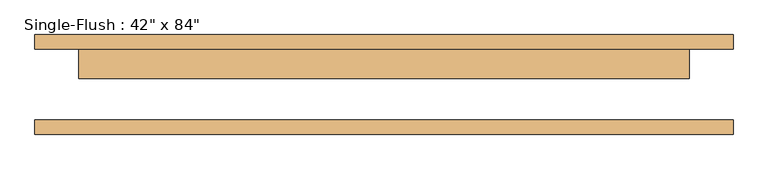
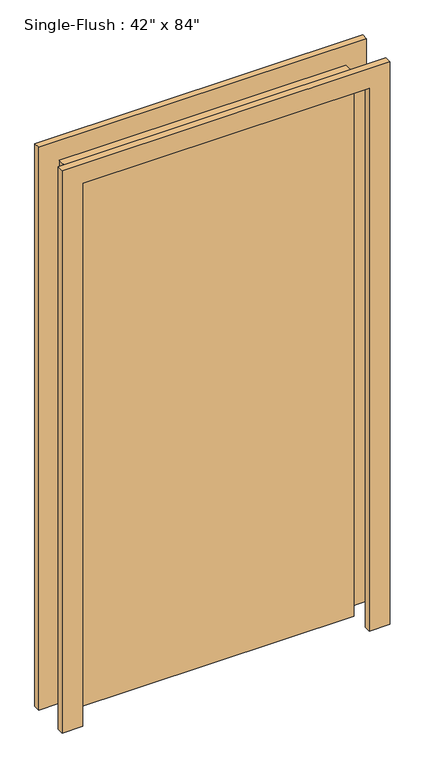
"""IFC4 building model written with IfcOpenShell, lengths in millimetres: door geometry."""

import ifcopenshell
import ifcopenshell.guid

model = None  # the IFC model being written
_history = None  # IfcOwnerHistory: only IFC2X3 demands one
_inside = {}  # id of a spatial element -> (the spatial element, [elements in it])
_under = {}  # id of a project, library or spatial element -> (it, [spatial elements below it])
_declared = {}  # id of a project -> (the project, [libraries it declares])
_typed = {}  # id of a type object -> (the type object, [elements of that type])
_made_of = {}  # id of a material, layer set ... -> (it, [elements and type objects made of it])


def new_model(schema):
    """Start an empty IFC model of exactly this schema.

    Asked for "IFC4X3", IfcOpenShell would pick the latest addendum, in which some entities
    have other attributes; the version numbers below select the first issue.
    IFC2X3 requires an IfcOwnerHistory on every rooted entity: one is made here for all.
    """
    global model, _history
    if schema == "IFC4X3":
        model = ifcopenshell.file(schema_version=(4, 3, 0, 0))
    else:
        model = ifcopenshell.file(schema=schema)
    _inside.clear()
    _under.clear()
    _declared.clear()
    _typed.clear()
    _made_of.clear()
    _history = None
    if model.schema == "IFC2X3":
        org = make("IfcOrganization", Name="unknown")
        user = make(
            "IfcPersonAndOrganization",
            ThePerson=make("IfcPerson", FamilyName="unknown"),
            TheOrganization=org,
        )
        app = make(
            "IfcApplication",
            ApplicationDeveloper=org,
            Version="unknown",
            ApplicationFullName="unknown",
            ApplicationIdentifier="unknown",
        )
        _history = make(
            "IfcOwnerHistory",
            OwningUser=user,
            OwningApplication=app,
            ChangeAction="ADDED",
            CreationDate=0,
        )
    return model


def make(cls, **values):
    """One entity of the class cls with the attributes given. An attribute that is None is left unset."""
    return model.create_entity(
        cls, **{name: value for name, value in values.items() if value is not None}
    )


def rooted(cls, **values):
    """An entity with a GlobalId (a new one), such as an element, a storey or a relation."""
    return make(cls, GlobalId=ifcopenshell.guid.new(), OwnerHistory=_history, **values)


def si_unit(unit_type, name, prefix=None):
    """IfcSIUnit, for example si_unit("LENGTHUNIT", "METRE", prefix="MILLI")."""
    return make("IfcSIUnit", UnitType=unit_type, Prefix=prefix, Name=name)


def assignment(units):
    """IfcUnitAssignment: the units of a project."""
    return None if units is None else make("IfcUnitAssignment", Units=units)


def point(xyz):
    """IfcCartesianPoint."""
    return None if xyz is None else make("IfcCartesianPoint", Coordinates=xyz)


def direction(xyz):
    """IfcDirection."""
    return None if xyz is None else make("IfcDirection", DirectionRatios=xyz)


def frame(location, z_axis=None, x_axis=None):
    """IfcAxis2Placement3D, a coordinate frame: its origin and axes. An axis left out is left unset."""
    return make(
        "IfcAxis2Placement3D",
        Location=point(location),
        Axis=direction(z_axis),
        RefDirection=direction(x_axis),
    )


def origin():
    """The frame at (0, 0, 0) with its axes left unset."""
    return frame((0.0, 0.0, 0.0))


def origin_with_axes():
    """The frame at (0, 0, 0) with the z axis (0, 0, 1) and the x axis (1, 0, 0) written out."""
    return frame((0.0, 0.0, 0.0), z_axis=(0.0, 0.0, 1.0), x_axis=(1.0, 0.0, 0.0))


def place(relative_to, where):
    """IfcLocalPlacement: puts the frame where relative to a parent placement (None: the world)."""
    return make(
        "IfcLocalPlacement", PlacementRelTo=relative_to, RelativePlacement=where
    )


def context(
    kind, dimensions, precision=None, world=None, true_north=None, identifier=None
):
    """IfcGeometricRepresentationContext, for example the 3D "Model" context."""
    return make(
        "IfcGeometricRepresentationContext",
        ContextIdentifier=identifier,
        ContextType=kind,
        CoordinateSpaceDimension=dimensions,
        Precision=precision,
        WorldCoordinateSystem=world,
        TrueNorth=true_north,
    )


def project(units=None, contexts=None):
    """IfcProject with its units and contexts."""
    return rooted(
        "IfcProject",
        Name="project",
        RepresentationContexts=contexts,
        UnitsInContext=assignment(units),
    )


def spatial(cls, under=None, at=None, **own):
    """A site, building, storey or space (cls), placed at a placement, below another one or the project."""
    s = rooted(cls, ObjectPlacement=at, **own)
    if under is not None:
        _under.setdefault(under.id(), (under, []))[1].append(s)
    return s


def polyline(points):
    """IfcPolyline through the points."""
    return make("IfcPolyline", Points=[point(p) for p in points])


def outline(outer, holes=None, kind="AREA"):
    """IfcArbitraryClosedProfileDef: a profile drawn as a closed curve; with holes, ...WithVoids."""
    if holes is None:
        return make("IfcArbitraryClosedProfileDef", ProfileType=kind, OuterCurve=outer)
    return make(
        "IfcArbitraryProfileDefWithVoids",
        ProfileType=kind,
        OuterCurve=outer,
        InnerCurves=holes,
    )


def extrude(swept, where, along, depth):
    """IfcExtrudedAreaSolid: the profile swept, set in the frame where, extruded along a direction by depth."""
    return make(
        "IfcExtrudedAreaSolid",
        SweptArea=swept,
        Position=where,
        ExtrudedDirection=direction(along),
        Depth=depth,
    )


def shape(context_of_items, identifier, shape_type, items):
    """IfcShapeRepresentation: the items that make up one representation, for example the "Body"."""
    return make(
        "IfcShapeRepresentation",
        ContextOfItems=context_of_items,
        RepresentationIdentifier=identifier,
        RepresentationType=shape_type,
        Items=items,
    )


def source(mapping_origin, context_of_items, identifier, shape_type, items):
    """IfcRepresentationMap: a shape defined once, which mapped items show again and again."""
    return make(
        "IfcRepresentationMap",
        MappingOrigin=mapping_origin,
        MappedRepresentation=shape(context_of_items, identifier, shape_type, items),
    )


def transform(
    local_origin,
    x_axis=None,
    y_axis=None,
    z_axis=None,
    scale=None,
    scale2=None,
    scale3=None,
    uniform=True,
):
    """IfcCartesianTransformationOperator3D, or its non-uniform kind. x_axis, y_axis, z_axis: its Axis1, 2, 3."""
    if uniform:
        return make(
            "IfcCartesianTransformationOperator3D",
            Axis1=direction(x_axis),
            Axis2=direction(y_axis),
            LocalOrigin=point(local_origin),
            Scale=scale,
            Axis3=direction(z_axis),
        )
    return make(
        "IfcCartesianTransformationOperator3DnonUniform",
        Axis1=direction(x_axis),
        Axis2=direction(y_axis),
        LocalOrigin=point(local_origin),
        Scale=scale,
        Axis3=direction(z_axis),
        Scale2=scale2,
        Scale3=scale3,
    )


def mapped(mapping_source, mapping_target):
    """IfcMappedItem: shows the shape of a source again, moved by a transform."""
    return make(
        "IfcMappedItem", MappingSource=mapping_source, MappingTarget=mapping_target
    )


def made_of(thing, what):
    """Note that an element or type object is made of a material, layer set ...; save() writes the relation."""
    if what is not None:
        _made_of.setdefault(what.id(), (what, []))[1].append(thing)
    return thing


def element(
    cls,
    number,
    at=None,
    inside=None,
    cuts=None,
    type_object=None,
    material=None,
    context=None,
    identifier="Body",
    shape_type=None,
    held_by="IfcProductDefinitionShape",
    body=None,
    shapes=None,
    **own,
):
    """One element of the class cls, such as IfcWall. Its Tag is "e" and its number.

    at: its placement. inside: the storey or other place that contains it. cuts: it is an
    opening in that element (IfcRelVoidsElement). A single representation is given by context,
    identifier, shape_type and body (its items); several are given by shapes. held_by: the class
    of the entity that holds the representations. save() writes the other relations.
    """
    e = rooted(cls, Tag="e%d" % number, ObjectPlacement=at, **own)
    if body is not None:
        shapes = [shape(context, identifier, shape_type, body)]
    if shapes is not None:
        e.Representation = make(held_by, Representations=shapes)
    if inside is not None:
        _inside.setdefault(inside.id(), (inside, []))[1].append(e)
    if cuts is not None:
        rooted(
            "IfcRelVoidsElement", RelatingBuildingElement=cuts, RelatedOpeningElement=e
        )
    if type_object is not None:
        _typed.setdefault(type_object.id(), (type_object, []))[1].append(e)
    return made_of(e, material)


def aggregate(whole, parts):
    """IfcRelAggregates: a whole, such as a stair, and the parts it consists of."""
    return rooted("IfcRelAggregates", RelatingObject=whole, RelatedObjects=parts)


def save(model, path):
    """Write the relations noted so far, then the file.

    IfcRelAggregates (storeys below a building ...), IfcRelContainedInSpatialStructure (elements
    in a storey), IfcRelDefinesByType, IfcRelAssociatesMaterial and IfcRelDeclares: one each for
    every whole, place, type object, material and project.
    """
    for whole, parts in _under.values():
        aggregate(whole, parts)
    for where, things in _inside.values():
        rooted(
            "IfcRelContainedInSpatialStructure",
            RelatedElements=things,
            RelatingStructure=where,
        )
    for kind, things in _typed.values():
        rooted("IfcRelDefinesByType", RelatedObjects=things, RelatingType=kind)
    for what, things in _made_of.values():
        rooted("IfcRelAssociatesMaterial", RelatedObjects=things, RelatingMaterial=what)
    for by, libraries in _declared.values():
        rooted("IfcRelDeclares", RelatingContext=by, RelatedDefinitions=libraries)
    model.write(path)


def door_af0cb62c(model_context):
    return source(origin(), model_context, "Body", "SweptSolid", [
        extrude(outline(polyline([(2209.8, -609.6), (0.0, -609.6), (0.0, -533.4), (2133.6, -533.4), (2133.6, 533.4), (0.0, 533.4), (0.0, 609.6), (2209.8, 609.6), (2209.8, -609.6)])), frame((0.0, 61.9125, 0.0), z_axis=(0.0, 1.0, 0.0), x_axis=(0.0, 0.0, 1.0)), (0.0, 0.0, 1.0), 25.4),
        extrude(outline(polyline([(2209.8, 609.6), (2209.8, -609.6), (0.0, -609.6), (0.0, -533.4), (2133.6, -533.4), (2133.6, 533.4), (0.0, 533.4), (0.0, 609.6), (2209.8, 609.6)])), frame((0.0, -87.3125, 0.0), z_axis=(0.0, 1.0, 0.0), x_axis=(0.0, 0.0, 1.0)), (0.0, 0.0, 1.0), 25.4),
        extrude(outline(polyline([(533.4, 11.1125), (-533.4, 11.1125), (-533.4, 61.9125), (533.4, 61.9125), (533.4, 11.1125)])), origin_with_axes(), (0.0, 0.0, 1.0), 2133.6),
    ])


if __name__ == "__main__":
    model = new_model("IFC4")
    model_context = context("Model", 3, world=origin())
    ifc_project = project(units=[si_unit("LENGTHUNIT", "METRE", prefix="MILLI")], contexts=[model_context])
    site = spatial("IfcSite", under=ifc_project)
    building = spatial("IfcBuilding", under=site)
    placement = place(None, origin())
    door_shape = door_af0cb62c(model_context)
    element("IfcDoor", 1, ObjectType="Single-Flush : 42\" x 84\"", at=placement, inside=building, context=model_context, shape_type="MappedRepresentation", body=[
        mapped(door_shape, transform((0.0, 0.0, 0.0), x_axis=(1.0, 0.0, 0.0), y_axis=(0.0, 1.0, 0.0), z_axis=(0.0, 0.0, 1.0))),
    ])
    save(model, "model.ifc")

# Revit data of these elements
# Type "Single-Flush : 42\" x 84\""
#   Type Mark = "9"
#   Construction Type = "B"
#   Assembly Code = "C1020"
#   Thickness = 0' - 2"
#   Height = 7' - 0"
#   Trim Projection Ext = 0' - 1"
#   Trim Projection Int = 0' - 1"
#   Trim Width = 0' - 3"
#   Width = 3' - 6"
#   Door Material = Door - Panel
#   Frame Material = Door - Frame
#   Function = (empty or 0)
#   Wall Closure = (empty or 0)
# Element 1 (IfcDoor, "Single-Flush : 42\" x 84\"")
#   Materials on its faces: "Door - Frame", "Door - Panel"
# Materials
#   "Door - Panel": class "Wood", colour RGB 210 159 95, transparency 0
#   "Door - Frame": class "Miscellaneous", colour RGB 118 70 51, transparency 0
